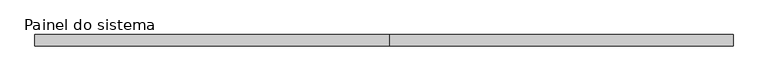
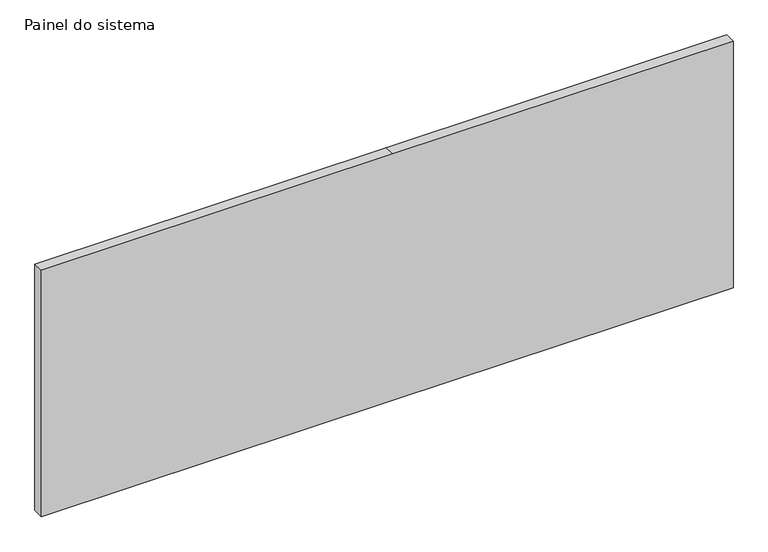
"""IFC4 building model written with IfcOpenShell, lengths in millimetres: plate geometry, Painel do sistema : Envidraçado."""

from ifc_helpers import new_model, si_unit, frame, origin, place, context, project, spatial, polyline, outline, extrude, source, transform, mapped, element, save


def painel_do_sistema_e8bc62b3(model_context):
    return source(origin(), model_context, "Body", "SweptSolid", [
        extrude(outline(polyline([(0.0, -783.4833334), (0.0, 12.4999998), (0.0, 783.4833334), (590.0, 783.4833334), (590.0, 12.4999998), (590.0, -783.4833334), (0.0, -783.4833334)])), frame((0.0, -49.5, 0.0), z_axis=(0.0, 1.0, 0.0), x_axis=(0.0, 0.0, 1.0)), (0.0, 0.0, 1.0), 25.0),
    ])


if __name__ == "__main__":
    model = new_model("IFC4")
    model_context = context("Model", 3, world=origin())
    ifc_project = project(units=[si_unit("LENGTHUNIT", "METRE", prefix="MILLI")], contexts=[model_context])
    site = spatial("IfcSite", under=ifc_project)
    building = spatial("IfcBuilding", under=site)
    placement = place(None, origin())
    painel_do_sistema_shape = painel_do_sistema_e8bc62b3(model_context)
    element("IfcPlate", 1, ObjectType="Painel do sistema : Envidraçado", at=placement, inside=building, context=model_context, shape_type="MappedRepresentation", body=[
        mapped(painel_do_sistema_shape, transform((0.0, 0.0, 0.0), x_axis=(1.0, 0.0, 0.0), y_axis=(0.0, 1.0, 0.0), z_axis=(0.0, 0.0, 1.0))),
    ])
    save(model, "model.ifc")

# Revit data of these elements
# Type "Painel do sistema : Envidraçado"
#   Construction Type Id = "GSP4R"
#   Analytic Construction = "Vidraça única Pilkington 1/8 pol"
#   Visual Light Transmittance = 0.9
#   Solar Heat Gain Coefficient = 0.86
#   Heat Transfer Coefficient (U) = 6.7069 W/(m²·K)
# Element 1 (IfcPlate, "Painel do sistema : Envidraçado")
#   Materials on its faces: ".VIDRO GENÉRICO"
# Materials
#   ".VIDRO GENÉRICO": class ".CC_VIDRO", colour RGB 0 128 192, transparency 0.9, Description = "Vidro comum", Cost = 0
